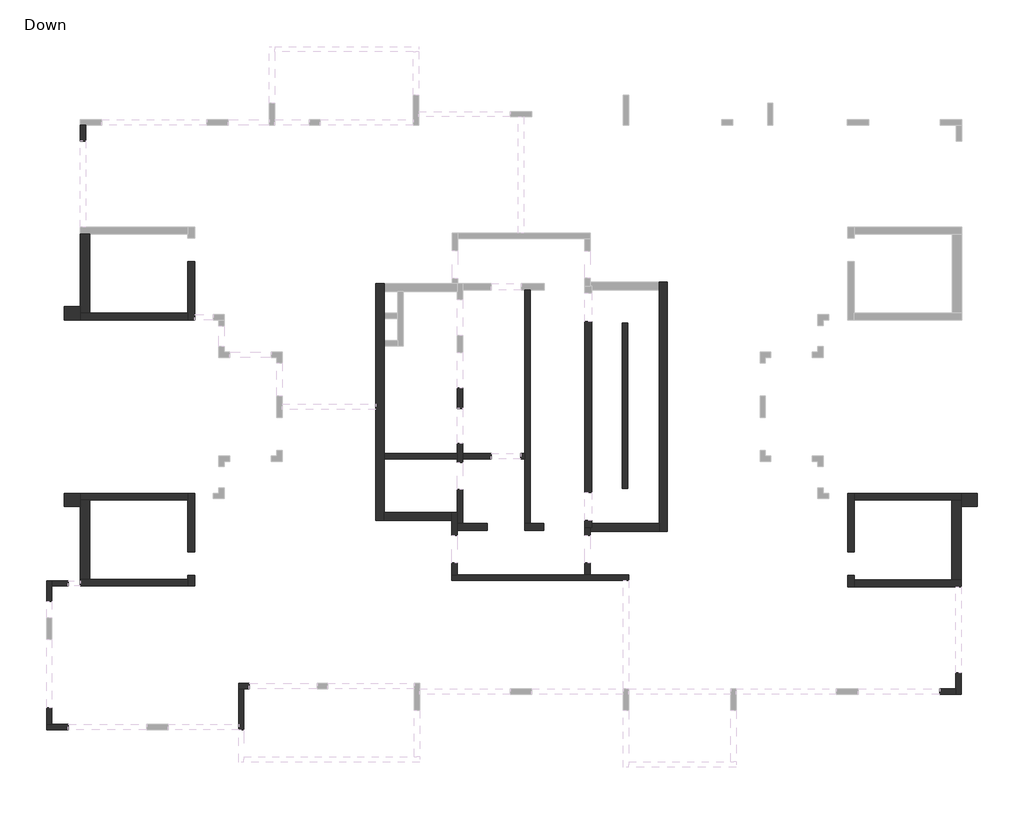
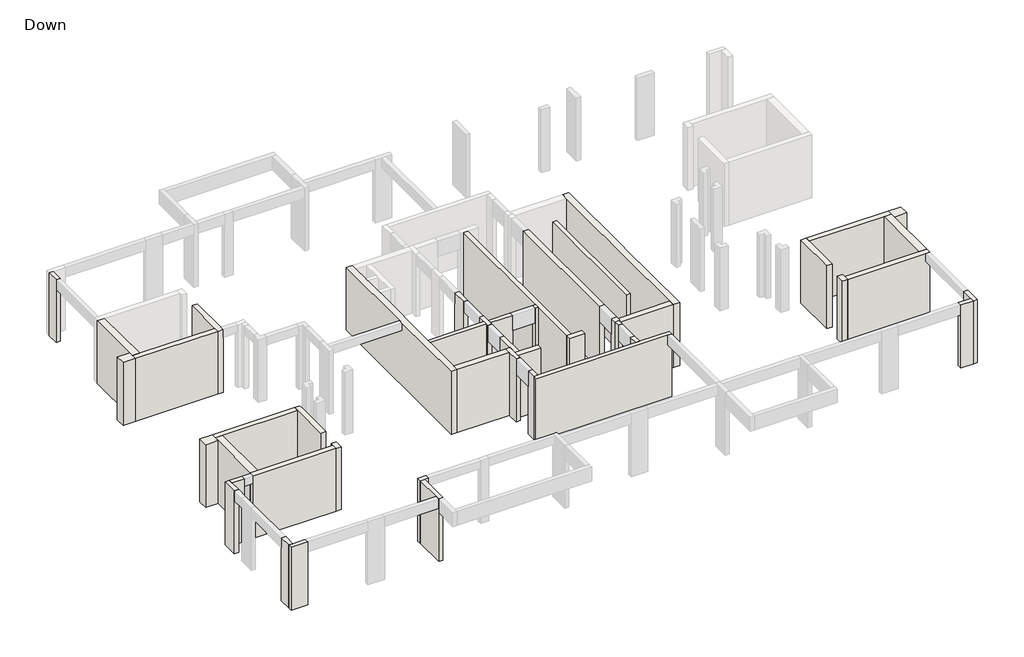
# One storey, part 1 of 3: 46 walls.
"""IFC4 building model written with IfcOpenShell, lengths in millimetres."""

from ifc_helpers import new_model, si_unit, origin, origin_with_axes, place, context, project, spatial, polyline, outline, extrude, faceted_brep, element, save

model = new_model("IFC4")

# Units and contexts
model_context = context("Model", 3, world=origin())
ifc_project = project(units=[si_unit("LENGTHUNIT", "METRE", prefix="MILLI")], contexts=[model_context])

# Site, building, storey
site = spatial("IfcSite", under=ifc_project)
building = spatial("IfcBuilding", under=site)
storey = spatial("IfcBuildingStorey", under=building, Name="Down", Elevation=0.0)

# Walls
placement = place(None, origin())
element("IfcWall", 1, ObjectType="20", at=placement, inside=storey, context=model_context, shape_type="Brep", body=[
    faceted_brep([(-16152.3851738, 8714.1448811, 0.0), (-16152.3851738, 8125.9123109, 0.0), (-16152.3851738, 8125.9123109, 2700.0), (-16152.3851738, 8125.9123109, 3200.0), (-16152.3851738, 8714.1448811, 3200.0), (-15952.3851738, 8714.1448811, 0.0), (-15952.3851738, 8714.1448811, 3020.0), (-15952.3851738, 8714.1448811, 3200.0), (-15952.3851738, 8125.9123109, 3200.0), (-15952.3851738, 8125.9123109, 2700.0), (-15952.3851738, 8125.9123109, 0.0)], [[[0, 1, 2, 3, 4]], [[5, 6, 7, 8, 9, 10]], [[1, 0, 5, 10]], [[3, 2, 1, 10, 9, 8]], [[4, 3, 8, 7]], [[0, 4, 7, 6, 5]]]),
])
element("IfcWall", 2, ObjectType="20", at=placement, inside=storey, context=model_context, shape_type="Brep", body=[
    faceted_brep([(-2227.8189264, -1013.9530422, 0.0), (-2227.8189264, -1753.9530422, 0.0), (-2227.8189264, -1753.9530422, 2670.0), (-2227.8189264, -1753.9530422, 3200.0), (-2227.8189264, -1013.9530422, 3200.0), (-2227.8189264, -1013.9530422, 2670.0), (-2027.8189264, -1013.9530422, 0.0), (-2027.8189264, -1013.9530422, 2670.0), (-2027.8189264, -1013.9530422, 3020.0), (-2027.8189264, -1013.9530422, 3200.0), (-2027.8189264, -1753.9530422, 3200.0), (-2027.8189264, -1753.9530422, 3020.0), (-2027.8189264, -1753.9530422, 2670.0), (-2027.8189264, -1753.9530422, 0.0), (-2032.8189264, -1753.9530422, 3200.0), (-2032.8189264, -1013.9530422, 3200.0)], [[[0, 1, 2, 3, 4, 5]], [[6, 7, 8, 9, 10, 11, 12, 13]], [[1, 0, 6, 13]], [[3, 2, 1, 13, 12, 11, 10, 14]], [[4, 3, 14, 10, 9, 15]], [[0, 5, 4, 15, 9, 8, 7, 6]]]),
])
element("IfcWall", 3, ObjectType="20", at=placement, inside=storey, context=model_context, shape_type="Brep", body=[
    faceted_brep([(-2227.8189264, -3053.9530422, 0.0), (-2227.8189264, -3433.9530422, 0.0), (-2227.8189264, -3633.9530422, 0.0), (-2227.8189264, -3753.9530422, 0.0), (-2227.8189264, -3753.9530422, 2420.0), (-2227.8189264, -3753.9530422, 3200.0), (-2227.8189264, -3633.9530422, 3200.0), (-2227.8189264, -3433.9530422, 3200.0), (-2227.8189264, -3053.9530422, 3200.0), (-2227.8189264, -3053.9530422, 2670.0), (-2027.8189264, -3053.9530422, 0.0), (-2027.8189264, -3053.9530422, 2670.0), (-2027.8189264, -3053.9530422, 3020.0), (-2027.8189264, -3053.9530422, 3200.0), (-2027.8189264, -3433.9530422, 3200.0), (-2027.8189264, -3633.9530422, 3200.0), (-2027.8189264, -3753.9530422, 3200.0), (-2027.8189264, -3753.9530422, 2420.0), (-2027.8189264, -3753.9530422, 0.0), (-2027.8189264, -3633.9530422, 0.0), (-2027.8189264, -3433.9530422, 0.0), (-2032.8189264, -3053.9530422, 3200.0)], [[[0, 1, 2, 3, 4, 5, 6, 7, 8, 9]], [[10, 11, 12, 13, 14, 15, 16, 17, 18, 19, 20]], [[3, 2, 1, 0, 10, 20, 19, 18]], [[5, 4, 3, 18, 17, 16]], [[8, 7, 6, 5, 16, 15, 14, 13, 21]], [[0, 9, 8, 21, 13, 12, 11, 10]]]),
])
element("IfcWall", 4, ObjectType="20", at=placement, inside=storey, context=model_context, shape_type="Brep", body=[
    faceted_brep([(-2027.8189264, -3633.9530422, 0.0), (-967.8189264, -3633.9530422, 0.0), (-967.8189264, -3633.9530422, 2420.0), (-967.8189264, -3633.9530422, 3200.0), (-2027.8189264, -3633.9530422, 3200.0), (-2027.8189264, -3633.9530422, 3020.0), (-2027.8189264, -3433.9530422, 0.0), (-2027.8189264, -3433.9530422, 3020.0), (-2027.8189264, -3433.9530422, 3200.0), (-967.8189264, -3433.9530422, 3200.0), (-967.8189264, -3433.9530422, 2420.0), (-967.8189264, -3433.9530422, 0.0)], [[[0, 1, 2, 3, 4, 5]], [[6, 7, 8, 9, 10, 11]], [[1, 0, 6, 11]], [[3, 2, 1, 11, 10, 9]], [[4, 3, 9, 8]], [[0, 5, 4, 8, 7, 6]]]),
])
element("IfcWall", 5, ObjectType="20", at=placement, inside=storey, context=model_context, shape_type="SweptSolid", body=[
    extrude(outline(polyline([(-4927.8189264, -3433.9530422), (-2227.8189264, -3433.9530422), (-2227.8189264, -3633.9530422), (-4927.8189264, -3633.9530422), (-4927.8189264, -3433.9530422)])), origin_with_axes(), (0.0, 0.0, 1.0), 3200.0),
])
element("IfcWall", 6, ObjectType="20", at=placement, inside=storey, context=model_context, shape_type="Brep", body=[
    faceted_brep([(272.1810736, -3433.9530422, 0.0), (122.0171251, -3433.9530422, 0.0), (122.0171251, -3433.9530422, 2420.0), (122.0171251, -3433.9530422, 3200.0), (272.1810736, -3433.9530422, 3200.0), (272.1810736, -3633.9530422, 0.0), (272.1810736, -3633.9530422, 3020.0), (272.1810736, -3633.9530422, 3200.0), (122.0171251, -3633.9530422, 3200.0), (122.0171251, -3633.9530422, 2420.0), (122.0171251, -3633.9530422, 0.0)], [[[0, 1, 2, 3, 4]], [[5, 6, 7, 8, 9, 10]], [[1, 0, 5, 10]], [[3, 2, 1, 10, 9, 8]], [[4, 3, 8, 7]], [[0, 4, 7, 6, 5]]]),
])
element("IfcWall", 7, ObjectType="20", at=placement, inside=storey, context=model_context, shape_type="Brep", body=[
    faceted_brep([(472.1810736, -6018.9082421, 0.0), (472.1810736, 2608.8247791, 0.0), (472.1810736, 2608.8247791, 3020.0), (472.1810736, 2608.8247791, 3200.0), (472.1810736, -6018.9082421, 3200.0), (472.1810736, -6018.9082421, 3020.0), (272.1810736, -6018.9082421, 0.0), (272.1810736, -6018.9082421, 3200.0), (272.1810736, -3633.9530422, 3200.0), (272.1810736, -3433.9530422, 3200.0), (272.1810736, 2608.8247791, 3200.0), (272.1810736, 2608.8247791, 3020.0), (272.1810736, 2608.8247791, 0.0), (272.1810736, -3433.9530422, 0.0), (272.1810736, -3633.9530422, 0.0)], [[[0, 1, 2, 3, 4, 5]], [[6, 7, 8, 9, 10, 11, 12, 13, 14]], [[1, 0, 6, 14, 13, 12]], [[4, 3, 10, 9, 8, 7]], [[3, 2, 1, 12, 11, 10]], [[0, 5, 4, 7, 6]]]),
])
element("IfcWall", 8, ObjectType="20", at=placement, inside=storey, context=model_context, shape_type="SweptSolid", body=[
    extrude(outline(polyline([(4072.1544873, 1402.9570331), (4072.1544873, -4717.0429669), (3872.1544873, -4717.0429669), (3872.1544873, 1402.9570331), (4072.1544873, 1402.9570331)])), origin_with_axes(), (0.0, 0.0, 1.0), 3200.0),
])
element("IfcWall", 9, ObjectType="20", at=placement, inside=storey, context=model_context, shape_type="Brep", body=[
    faceted_brep([(2484.725333, -6161.1752209, 0.0), (2484.725333, -6451.1752209, 0.0), (2484.725333, -6451.1752209, 2420.0), (2484.725333, -6451.1752209, 3200.0), (2484.725333, -6161.1752209, 3200.0), (2684.725333, -6161.1752209, 0.0), (2684.725333, -6161.1752209, 3200.0), (2684.725333, -6311.1752209, 3200.0), (2684.725333, -6451.1752209, 3200.0), (2684.725333, -6451.1752209, 2420.0), (2684.725333, -6451.1752209, 0.0), (2684.725333, -6311.1752209, 0.0)], [[[0, 1, 2, 3, 4]], [[5, 6, 7, 8, 9, 10, 11]], [[1, 0, 5, 11, 10]], [[3, 2, 1, 10, 9, 8]], [[4, 3, 8, 7, 6]], [[0, 4, 6, 5]]]),
])
element("IfcWall", 10, ObjectType="20", at=placement, inside=storey, context=model_context, shape_type="Brep", body=[
    faceted_brep([(2484.725333, -7471.1752209, 0.0), (2484.725333, -7911.1752209, 0.0), (2484.725333, -7911.1752209, 3020.0), (2484.725333, -7911.1752209, 3200.0), (2484.725333, -7471.1752209, 3200.0), (2484.725333, -7471.1752209, 2420.0), (2684.725333, -7471.1752209, 0.0), (2684.725333, -7471.1752209, 2420.0), (2684.725333, -7471.1752209, 3200.0), (2684.725333, -7911.1752209, 3200.0), (2684.725333, -7911.1752209, 3020.0), (2684.725333, -7911.1752209, 0.0)], [[[0, 1, 2, 3, 4, 5]], [[6, 7, 8, 9, 10, 11]], [[1, 0, 6, 11]], [[4, 3, 9, 8]], [[0, 5, 4, 8, 7, 6]], [[3, 2, 1, 11, 10, 9]]]),
])
element("IfcWall", 11, ObjectType="20", at=placement, inside=storey, context=model_context, shape_type="Brep", body=[
    faceted_brep([(4107.8539459, -7911.1752209, 0.0), (2684.725333, -7911.1752209, 0.0), (2484.725333, -7911.1752209, 0.0), (-2224.4804119, -7911.1752209, 0.0), (-2424.4804119, -7911.1752209, 0.0), (-2424.4804119, -7911.1752209, 3200.0), (-2224.4804119, -7911.1752209, 3200.0), (2484.725333, -7911.1752209, 3200.0), (2684.725333, -7911.1752209, 3200.0), (4107.8539459, -7911.1752209, 3200.0), (4107.8539459, -7911.1752209, 3020.0), (4107.8539459, -8111.1752209, 0.0), (4107.8539459, -8111.1752209, 3200.0), (3907.8539459, -8111.1752209, 3200.0), (-2424.4804119, -8111.1752209, 3200.0), (-2424.4804119, -8111.1752209, 3020.0), (-2424.4804119, -8111.1752209, 0.0)], [[[0, 1, 2, 3, 4, 5, 6, 7, 8, 9, 10]], [[11, 12, 13, 14, 15, 16]], [[4, 3, 2, 1, 0, 11, 16]], [[9, 8, 7, 6, 5, 14, 13, 12]], [[0, 10, 9, 12, 11]], [[5, 4, 16, 15, 14]]]),
])
element("IfcWall", 12, ObjectType="20", at=placement, inside=storey, context=model_context, shape_type="Brep", body=[
    faceted_brep([(-2224.4804119, -7911.1752209, 0.0), (-2224.4804119, -7466.1752209, 0.0), (-2224.4804119, -7466.1752209, 2420.0), (-2224.4804119, -7466.1752209, 3200.0), (-2224.4804119, -7911.1752209, 3200.0), (-2224.4804119, -7911.1752209, 3020.0), (-2424.4804119, -7911.1752209, 0.0), (-2424.4804119, -7911.1752209, 3200.0), (-2424.4804119, -7466.1752209, 3200.0), (-2424.4804119, -7466.1752209, 2420.0), (-2424.4804119, -7466.1752209, 0.0)], [[[0, 1, 2, 3, 4, 5]], [[6, 7, 8, 9, 10]], [[1, 0, 6, 10]], [[3, 2, 1, 10, 9, 8]], [[4, 3, 8, 7]], [[0, 5, 4, 7, 6]]]),
])
element("IfcWall", 13, ObjectType="20", at=placement, inside=storey, context=model_context, shape_type="Brep", body=[
    faceted_brep([(-2224.4804119, -6461.1752209, 0.0), (-2224.4804119, -6261.1752209, 0.0), (-2224.4804119, -6011.1752209, 0.0), (-2224.4804119, -5601.1752209, 0.0), (-2224.4804119, -5601.1752209, 3200.0), (-2224.4804119, -6011.1752209, 3200.0), (-2224.4804119, -6261.1752209, 3200.0), (-2224.4804119, -6461.1752209, 3200.0), (-2224.4804119, -6461.1752209, 2420.0), (-2424.4804119, -6461.1752209, 0.0), (-2424.4804119, -6461.1752209, 2420.0), (-2424.4804119, -6461.1752209, 3200.0), (-2424.4804119, -5901.1752209, 3200.0), (-2424.4804119, -5601.1752209, 3200.0), (-2424.4804119, -5601.1752209, 0.0), (-2424.4804119, -5901.1752209, 0.0), (-2227.8189264, -5601.1752209, 0.0), (-2227.8189264, -5601.1752209, 3200.0)], [[[0, 1, 2, 3, 4, 5, 6, 7, 8]], [[9, 10, 11, 12, 13, 14, 15]], [[3, 2, 1, 0, 9, 15, 14, 16]], [[7, 6, 5, 4, 17, 13, 12, 11]], [[0, 8, 7, 11, 10, 9]], [[4, 3, 16, 14, 13, 17]]]),
])
element("IfcWall", 14, ObjectType="20", at=placement, inside=storey, context=model_context, shape_type="Brep", body=[
    faceted_brep([(-2227.8189264, -4756.1752209, 3200.0), (-2227.8189264, -4756.1752209, 2420.0), (-2227.8189264, -4756.1752209, 0.0), (-2227.8189264, -5601.1752209, 0.0), (-2227.8189264, -5601.1752209, 3200.0), (-2027.8189264, -6011.1752209, 0.0), (-2027.8189264, -4756.1752209, 0.0), (-2027.8189264, -4756.1752209, 2420.0), (-2027.8189264, -4756.1752209, 3200.0), (-2027.8189264, -6011.1752209, 3200.0), (-2027.8189264, -6011.1752209, 3020.0), (-2224.4804119, -6011.1752209, 0.0), (-2224.4804119, -5601.1752209, 0.0), (-2224.4804119, -5601.1752209, 3200.0), (-2224.4804119, -6011.1752209, 3200.0)], [[[0, 1, 2, 3, 4]], [[5, 6, 7, 8, 9, 10]], [[6, 5, 11, 12, 3, 2]], [[9, 8, 0, 4, 13, 14]], [[2, 1, 0, 8, 7, 6]], [[5, 10, 9, 14, 11]], [[13, 12, 11, 14]], [[12, 13, 4, 3]]]),
])
element("IfcWall", 15, ObjectType="20", at=placement, inside=storey, context=model_context, shape_type="Brep", body=[
    faceted_brep([(16190.4478267, -11524.2691374, 0.0), (16190.4478267, -12124.2691374, 0.0), (16190.4478267, -12324.2691374, 0.0), (16190.4478267, -12324.2691374, 3200.0), (16190.4478267, -12124.2691374, 3200.0), (16190.4478267, -11524.2691374, 3200.0), (16190.4478267, -11524.2691374, 2800.0), (16390.4478267, -11524.2691374, 0.0), (16390.4478267, -11524.2691374, 2800.0), (16390.4478267, -11524.2691374, 3200.0), (16390.4478267, -12324.2691374, 3200.0), (16390.4478267, -12324.2691374, 0.0)], [[[0, 1, 2, 3, 4, 5, 6]], [[7, 8, 9, 10, 11]], [[2, 1, 0, 7, 11]], [[5, 4, 3, 10, 9]], [[0, 6, 5, 9, 8, 7]], [[3, 2, 11, 10]]]),
])
element("IfcWall", 16, ObjectType="20", at=placement, inside=storey, context=model_context, shape_type="Brep", body=[
    faceted_brep([(16190.4478267, -12124.2691374, 0.0), (15592.9268131, -12124.2691374, 0.0), (15592.9268131, -12124.2691374, 2700.0), (15592.9268131, -12124.2691374, 3200.0), (16190.4478267, -12124.2691374, 3200.0), (16190.4478267, -12124.2691374, 3020.0), (16190.4478267, -12324.2691374, 0.0), (16190.4478267, -12324.2691374, 3200.0), (15592.9268131, -12324.2691374, 3200.0), (15592.9268131, -12324.2691374, 2700.0), (15592.9268131, -12324.2691374, 0.0)], [[[0, 1, 2, 3, 4, 5]], [[6, 7, 8, 9, 10]], [[1, 0, 6, 10]], [[3, 2, 1, 10, 9, 8]], [[4, 3, 8, 7]], [[0, 5, 4, 7, 6]]]),
])
element("IfcWall", 17, ObjectType="20", at=placement, inside=storey, context=model_context, shape_type="Brep", body=[
    faceted_brep([(-9913.9547043, -11921.300832, 0.0), (-10303.9547043, -11921.300832, 0.0), (-10303.9547043, -11921.300832, 3020.0), (-10303.9547043, -11921.300832, 3200.0), (-9913.9547043, -11921.300832, 3200.0), (-9913.9547043, -11921.300832, 2800.0), (-9913.9547043, -12121.300832, 0.0), (-9913.9547043, -12121.300832, 2800.0), (-9913.9547043, -12121.300832, 3200.0), (-10103.9547043, -12121.300832, 3200.0), (-10303.9547043, -12121.300832, 3200.0), (-10303.9547043, -12121.300832, 0.0), (-10103.9547043, -12121.300832, 0.0)], [[[0, 1, 2, 3, 4, 5]], [[6, 7, 8, 9, 10, 11, 12]], [[1, 0, 6, 12, 11]], [[4, 3, 10, 9, 8]], [[0, 5, 4, 8, 7, 6]], [[3, 2, 1, 11, 10]]]),
])
element("IfcWall", 18, ObjectType="20", at=placement, inside=storey, context=model_context, shape_type="Brep", body=[
    faceted_brep([(-10303.9547043, -12121.300832, 0.0), (-10303.9547043, -13632.1139628, 0.0), (-10303.9547043, -13632.1139628, 2500.0), (-10303.9547043, -13632.1139628, 3200.0), (-10303.9547043, -13432.1139628, 3200.0), (-10303.9547043, -12121.300832, 3200.0), (-10103.9547043, -12121.300832, 0.0), (-10103.9547043, -12121.300832, 3020.0), (-10103.9547043, -12121.300832, 3200.0), (-10103.9547043, -13632.1139628, 3200.0), (-10103.9547043, -13632.1139628, 2500.0), (-10103.9547043, -13632.1139628, 0.0)], [[[0, 1, 2, 3, 4, 5]], [[6, 7, 8, 9, 10, 11]], [[1, 0, 6, 11]], [[3, 2, 1, 11, 10, 9]], [[5, 4, 3, 9, 8]], [[0, 5, 8, 7, 6]]]),
])
element("IfcWall", 19, ObjectType="20", at=placement, inside=storey, context=model_context, shape_type="Brep", body=[
    faceted_brep([(-16594.74029, -13432.1139628, 0.0), (-17194.74029, -13432.1139628, 0.0), (-17394.74029, -13432.1139628, 0.0), (-17394.74029, -13432.1139628, 3200.0), (-17194.74029, -13432.1139628, 3200.0), (-16594.74029, -13432.1139628, 3200.0), (-16594.74029, -13432.1139628, 2700.0), (-16594.74029, -13632.1139628, 0.0), (-16594.74029, -13632.1139628, 2700.0), (-16594.74029, -13632.1139628, 3200.0), (-17394.74029, -13632.1139628, 3200.0), (-17394.74029, -13632.1139628, 0.0)], [[[0, 1, 2, 3, 4, 5, 6]], [[7, 8, 9, 10, 11]], [[2, 1, 0, 7, 11]], [[5, 4, 3, 10, 9]], [[0, 6, 5, 9, 8, 7]], [[3, 2, 11, 10]]]),
])
element("IfcWall", 20, ObjectType="20", at=placement, inside=storey, context=model_context, shape_type="Brep", body=[
    faceted_brep([(-17194.74029, -13432.1139628, 0.0), (-17194.74029, -12822.7787814, 0.0), (-17194.74029, -12822.7787814, 2700.0), (-17194.74029, -12822.7787814, 3200.0), (-17194.74029, -13432.1139628, 3200.0), (-17194.74029, -13432.1139628, 3020.0), (-17394.74029, -13432.1139628, 0.0), (-17394.74029, -13432.1139628, 3200.0), (-17394.74029, -12822.7787814, 3200.0), (-17394.74029, -12822.7787814, 2700.0), (-17394.74029, -12822.7787814, 0.0)], [[[0, 1, 2, 3, 4, 5]], [[6, 7, 8, 9, 10]], [[1, 0, 6, 10]], [[3, 2, 1, 10, 9, 8]], [[4, 3, 8, 7]], [[0, 5, 4, 7, 6]]]),
])
element("IfcWall", 21, ObjectType="20", at=placement, inside=storey, context=model_context, shape_type="Brep", body=[
    faceted_brep([(-17194.74029, -8893.4441313, 0.0), (-17194.74029, -8327.5852261, 0.0), (-17194.74029, -8127.5852261, 0.0), (-17194.74029, -8127.5852261, 3200.0), (-17194.74029, -8327.5852261, 3200.0), (-17194.74029, -8893.4441313, 3200.0), (-17194.74029, -8893.4441313, 2700.0), (-17394.74029, -8893.4441313, 0.0), (-17394.74029, -8893.4441313, 2700.0), (-17394.74029, -8893.4441313, 3200.0), (-17394.74029, -8127.5852261, 3200.0), (-17394.74029, -8127.5852261, 0.0)], [[[0, 1, 2, 3, 4, 5, 6]], [[7, 8, 9, 10, 11]], [[2, 1, 0, 7, 11]], [[5, 4, 3, 10, 9]], [[0, 6, 5, 9, 8, 7]], [[3, 2, 11, 10]]]),
])
element("IfcWall", 22, ObjectType="20", at=placement, inside=storey, context=model_context, shape_type="Brep", body=[
    faceted_brep([(-17194.74029, -8327.5852261, 0.0), (-16589.4316206, -8327.5852261, 0.0), (-16589.4316206, -8327.5852261, 2800.0), (-16589.4316206, -8327.5852261, 3200.0), (-17194.74029, -8327.5852261, 3200.0), (-17194.74029, -8327.5852261, 3020.0), (-17194.74029, -8127.5852261, 0.0), (-17194.74029, -8127.5852261, 3200.0), (-16589.4316206, -8127.5852261, 3200.0), (-16589.4316206, -8127.5852261, 2800.0), (-16589.4316206, -8127.5852261, 0.0)], [[[0, 1, 2, 3, 4, 5]], [[6, 7, 8, 9, 10]], [[1, 0, 6, 10]], [[3, 2, 1, 10, 9, 8]], [[4, 3, 8, 7]], [[0, 5, 4, 7, 6]]]),
])
element("IfcWall", 23, ObjectType="25", at=placement, inside=storey, context=model_context, shape_type="Brep", body=[
    faceted_brep([(-12179.8186713, 3668.3687969, 0.0), (-12179.8186713, 1755.2784849, 0.0), (-12179.8186713, 1505.2784849, 0.0), (-12179.8186713, 1505.2784849, 3200.0), (-12179.8186713, 1755.2784849, 3200.0), (-12179.8186713, 3668.3687969, 3200.0), (-12179.8186713, 3668.3687969, 3020.0), (-11929.8186713, 3668.3687969, 0.0), (-11929.8186713, 3668.3687969, 3020.0), (-11929.8186713, 3668.3687969, 3200.0), (-11929.8186713, 1705.2784849, 3200.0), (-11929.8186713, 1505.2784849, 3200.0), (-11929.8186713, 1505.2784849, 2800.0), (-11929.8186713, 1505.2784849, 0.0)], [[[0, 1, 2, 3, 4, 5, 6]], [[7, 8, 9, 10, 11, 12, 13]], [[2, 1, 0, 7, 13]], [[5, 4, 3, 11, 10, 9]], [[0, 6, 5, 9, 8, 7]], [[3, 2, 13, 12, 11]]]),
])
element("IfcWall", 24, ObjectType="25", at=placement, inside=storey, context=model_context, shape_type="Brep", body=[
    faceted_brep([(-12179.8186713, 1755.2784849, 0.0), (-15802.3851738, 1755.2784849, 0.0), (-16152.3851738, 1755.2784849, 0.0), (-16152.3851738, 1755.2784849, 3200.0), (-15802.3851738, 1755.2784849, 3200.0), (-12179.8186713, 1755.2784849, 3200.0), (-12179.8186713, 1755.2784849, 3020.0), (-12179.8186713, 1505.2784849, 0.0), (-12179.8186713, 1505.2784849, 3200.0), (-16152.3851738, 1505.2784849, 3200.0), (-16152.3851738, 1505.2784849, 0.0)], [[[0, 1, 2, 3, 4, 5, 6]], [[7, 8, 9, 10]], [[2, 1, 0, 7, 10]], [[5, 4, 3, 9, 8]], [[0, 6, 5, 8, 7]], [[3, 2, 10, 9]]]),
])
element("IfcWall", 25, ObjectType="25", at=placement, inside=storey, context=model_context, shape_type="Brep", body=[
    faceted_brep([(2484.725333, -5901.1752209, 0.0), (2484.725333, -6161.1752209, 0.0), (2484.725333, -6161.1752209, 3200.0), (2484.725333, -5901.1752209, 3200.0), (2484.725333, -5901.1752209, 2420.0), (2734.725333, -5901.1752209, 0.0), (2734.725333, -5901.1752209, 2420.0), (2734.725333, -5901.1752209, 3200.0), (2734.725333, -6011.1752209, 3200.0), (2734.725333, -6161.1752209, 3200.0), (2734.725333, -6161.1752209, 0.0), (2734.725333, -6011.1752209, 0.0), (2684.725333, -6161.1752209, 0.0), (2684.725333, -6161.1752209, 3200.0)], [[[0, 1, 2, 3, 4]], [[5, 6, 7, 8, 9, 10, 11]], [[1, 0, 5, 11, 10, 12]], [[2, 1, 12, 10, 9, 13]], [[3, 2, 13, 9, 8, 7]], [[0, 4, 3, 7, 6, 5]]]),
])
element("IfcWall", 26, ObjectType="25", at=placement, inside=storey, context=model_context, shape_type="Brep", body=[
    faceted_brep([(-12179.8186713, -8077.5852261, 0.0), (-15802.3851738, -8077.5852261, 0.0), (-16152.3851738, -8077.5852261, 0.0), (-16152.3851738, -8077.5852261, 3200.0), (-15802.3851738, -8077.5852261, 3200.0), (-12179.8186713, -8077.5852261, 3200.0), (-12179.8186713, -8077.5852261, 3020.0), (-12179.8186713, -8327.5852261, 0.0), (-12179.8186713, -8327.5852261, 3200.0), (-16152.3851738, -8327.5852261, 3200.0), (-16152.3851738, -8327.5852261, 2800.0), (-16152.3851738, -8327.5852261, 0.0), (-16152.3851738, -8127.5852261, 3200.0)], [[[0, 1, 2, 3, 4, 5, 6]], [[7, 8, 9, 10, 11]], [[2, 1, 0, 7, 11]], [[5, 4, 3, 12, 9, 8]], [[0, 6, 5, 8, 7]], [[3, 2, 11, 10, 9, 12]]]),
])
element("IfcWall", 27, ObjectType="25", at=placement, inside=storey, context=model_context, shape_type="Brep", body=[
    faceted_brep([(-11929.8186713, -8327.5852261, 0.0), (-11929.8186713, -7927.5852261, 0.0), (-11929.8186713, -7927.5852261, 3020.0), (-11929.8186713, -7927.5852261, 3200.0), (-11929.8186713, -8327.5852261, 3200.0), (-11929.8186713, -8327.5852261, 3020.0), (-12179.8186713, -8327.5852261, 0.0), (-12179.8186713, -8327.5852261, 3200.0), (-12179.8186713, -8077.5852261, 3200.0), (-12179.8186713, -7927.5852261, 3200.0), (-12179.8186713, -7927.5852261, 3020.0), (-12179.8186713, -7927.5852261, 0.0), (-12179.8186713, -8077.5852261, 0.0)], [[[0, 1, 2, 3, 4, 5]], [[6, 7, 8, 9, 10, 11, 12]], [[1, 0, 6, 12, 11]], [[3, 2, 1, 11, 10, 9]], [[4, 3, 9, 8, 7]], [[0, 5, 4, 7, 6]]]),
])
element("IfcWall", 28, ObjectType="25", at=placement, inside=storey, context=model_context, shape_type="Brep", body=[
    faceted_brep([(-11929.8186713, -7056.2748812, 0.0), (-11929.8186713, -4893.1845693, 0.0), (-11929.8186713, -4893.1845693, 2800.0), (-11929.8186713, -4893.1845693, 3200.0), (-11929.8186713, -5093.1845693, 3200.0), (-11929.8186713, -7056.2748812, 3200.0), (-11929.8186713, -7056.2748812, 3020.0), (-12179.8186713, -7056.2748812, 0.0), (-12179.8186713, -7056.2748812, 3020.0), (-12179.8186713, -7056.2748812, 3200.0), (-12179.8186713, -5143.1845693, 3200.0), (-12179.8186713, -4893.1845693, 3200.0), (-12179.8186713, -4893.1845693, 0.0), (-12179.8186713, -5143.1845693, 0.0)], [[[0, 1, 2, 3, 4, 5, 6]], [[7, 8, 9, 10, 11, 12, 13]], [[1, 0, 7, 13, 12]], [[5, 4, 3, 11, 10, 9]], [[0, 6, 5, 9, 8, 7]], [[3, 2, 1, 12, 11]]]),
])
element("IfcWall", 29, ObjectType="25", at=placement, inside=storey, context=model_context, shape_type="Brep", body=[
    faceted_brep([(-12179.8186713, -4893.1845693, 0.0), (-16152.3851738, -4893.1845693, 0.0), (-16152.3851738, -4893.1845693, 3200.0), (-12179.8186713, -4893.1845693, 3200.0), (-12179.8186713, -5143.1845693, 0.0), (-12179.8186713, -5143.1845693, 3020.0), (-12179.8186713, -5143.1845693, 3200.0), (-15802.3851738, -5143.1845693, 3200.0), (-16152.3851738, -5143.1845693, 3200.0), (-16152.3851738, -5143.1845693, 0.0), (-15802.3851738, -5143.1845693, 0.0)], [[[0, 1, 2, 3]], [[4, 5, 6, 7, 8, 9, 10]], [[1, 0, 4, 10, 9]], [[3, 2, 8, 7, 6]], [[0, 3, 6, 5, 4]], [[2, 1, 9, 8]]]),
])
element("IfcWall", 30, ObjectType="25", at=placement, inside=storey, context=model_context, shape_type="Brep", body=[
    faceted_brep([(12437.8813243, -8347.5852261, 0.0), (16390.4478267, -8347.5852261, 0.0), (16390.4478267, -8347.5852261, 2800.0), (16390.4478267, -8347.5852261, 3200.0), (16190.4478267, -8347.5852261, 3200.0), (12437.8813243, -8347.5852261, 3200.0), (12437.8813243, -8097.5852261, 0.0), (12437.8813243, -8097.5852261, 3020.0), (12437.8813243, -8097.5852261, 3200.0), (16040.4478267, -8097.5852261, 3200.0), (16390.4478267, -8097.5852261, 3200.0), (16390.4478267, -8097.5852261, 0.0), (16040.4478267, -8097.5852261, 0.0)], [[[0, 1, 2, 3, 4, 5]], [[6, 7, 8, 9, 10, 11, 12]], [[1, 0, 6, 12, 11]], [[5, 4, 3, 10, 9, 8]], [[0, 5, 8, 7, 6]], [[3, 2, 1, 11, 10]]]),
])
element("IfcWall", 31, ObjectType="25", at=placement, inside=storey, context=model_context, shape_type="Brep", body=[
    faceted_brep([(12437.8813243, -8347.5852261, 0.0), (12437.8813243, -8097.5852261, 0.0), (12437.8813243, -7927.5852261, 0.0), (12437.8813243, -7927.5852261, 3020.0), (12437.8813243, -7927.5852261, 3200.0), (12437.8813243, -8097.5852261, 3200.0), (12437.8813243, -8347.5852261, 3200.0), (12187.8813243, -8347.5852261, 0.0), (12187.8813243, -8347.5852261, 3020.0), (12187.8813243, -8347.5852261, 3200.0), (12187.8813243, -7927.5852261, 3200.0), (12187.8813243, -7927.5852261, 3020.0), (12187.8813243, -7927.5852261, 0.0)], [[[0, 1, 2, 3, 4, 5, 6]], [[7, 8, 9, 10, 11, 12]], [[2, 1, 0, 7, 12]], [[4, 3, 2, 12, 11, 10]], [[6, 5, 4, 10, 9]], [[0, 6, 9, 8, 7]]]),
])
element("IfcWall", 32, ObjectType="25", at=placement, inside=storey, context=model_context, shape_type="Brep", body=[
    faceted_brep([(12437.8813243, -7056.2748812, 0.0), (12437.8813243, -5143.1845693, 0.0), (12437.8813243, -4893.1845693, 0.0), (12437.8813243, -4893.1845693, 3200.0), (12437.8813243, -5143.1845693, 3200.0), (12437.8813243, -7056.2748812, 3200.0), (12437.8813243, -7056.2748812, 3020.0), (12187.8813243, -7056.2748812, 0.0), (12187.8813243, -7056.2748812, 3020.0), (12187.8813243, -7056.2748812, 3200.0), (12187.8813243, -5093.1845693, 3200.0), (12187.8813243, -4893.1845693, 3200.0), (12187.8813243, -4893.1845693, 2800.0), (12187.8813243, -4893.1845693, 0.0)], [[[0, 1, 2, 3, 4, 5, 6]], [[7, 8, 9, 10, 11, 12, 13]], [[2, 1, 0, 7, 13]], [[5, 4, 3, 11, 10, 9]], [[0, 6, 5, 9, 8, 7]], [[3, 2, 13, 12, 11]]]),
])
element("IfcWall", 33, ObjectType="25", at=placement, inside=storey, context=model_context, shape_type="Brep", body=[
    faceted_brep([(12437.8813243, -5143.1845693, 0.0), (16040.4478267, -5143.1845693, 0.0), (16390.4478267, -5143.1845693, 0.0), (16390.4478267, -5143.1845693, 3200.0), (16040.4478267, -5143.1845693, 3200.0), (12437.8813243, -5143.1845693, 3200.0), (12437.8813243, -5143.1845693, 3020.0), (12437.8813243, -4893.1845693, 0.0), (12437.8813243, -4893.1845693, 3200.0), (16390.4478267, -4893.1845693, 3200.0), (16390.4478267, -4893.1845693, 0.0)], [[[0, 1, 2, 3, 4, 5, 6]], [[7, 8, 9, 10]], [[2, 1, 0, 7, 10]], [[5, 4, 3, 9, 8]], [[0, 6, 5, 8, 7]], [[3, 2, 10, 9]]]),
])
element("IfcWall", 34, ObjectType="25", at=placement, inside=storey, context=model_context, shape_type="Brep", body=[
    faceted_brep([(2484.725333, 1454.2743435, 0.0), (2484.725333, -4865.7256565, 0.0), (2484.725333, -4865.7256565, 2420.0), (2484.725333, -4865.7256565, 3200.0), (2484.725333, 1454.2743435, 3200.0), (2484.725333, 1454.2743435, 2420.0), (2734.725333, 1454.2743435, 0.0), (2734.725333, 1454.2743435, 2420.0), (2734.725333, 1454.2743435, 3200.0), (2734.725333, 1402.9570331, 3200.0), (2734.725333, -4865.7256565, 3200.0), (2734.725333, -4865.7256565, 2420.0), (2734.725333, -4865.7256565, 0.0)], [[[0, 1, 2, 3, 4, 5]], [[6, 7, 8, 9, 10, 11, 12]], [[1, 0, 6, 12]], [[3, 2, 1, 12, 11, 10]], [[4, 3, 10, 9, 8]], [[0, 5, 4, 8, 7, 6]]]),
])
element("IfcWall", 35, ObjectType="25", at=placement, inside=storey, context=model_context, shape_type="Brep", body=[
    faceted_brep([(-2224.4804119, -6261.1752209, 0.0), (-1124.4804119, -6261.1752209, 0.0), (-1124.4804119, -6261.1752209, 3020.0), (-1124.4804119, -6261.1752209, 3200.0), (-2224.4804119, -6261.1752209, 3200.0), (-2224.4804119, -6261.1752209, 3020.0), (-2224.4804119, -6011.1752209, 0.0), (-2224.4804119, -6011.1752209, 3200.0), (-2027.8189264, -6011.1752209, 3200.0), (-1124.4804119, -6011.1752209, 3200.0), (-1124.4804119, -6011.1752209, 3020.0), (-1124.4804119, -6011.1752209, 0.0), (-2027.8189264, -6011.1752209, 0.0)], [[[0, 1, 2, 3, 4, 5]], [[6, 7, 8, 9, 10, 11, 12]], [[1, 0, 6, 12, 11]], [[3, 2, 1, 11, 10, 9]], [[4, 3, 9, 8, 7]], [[0, 5, 4, 7, 6]]]),
])
element("IfcWall", 36, ObjectType="25", at=placement, inside=storey, context=model_context, shape_type="Brep", body=[
    faceted_brep([(974.071657, -6018.9082421, 0.0), (472.1810736, -6018.9082421, 0.0), (272.1810736, -6018.9082421, 0.0), (272.1810736, -6018.9082421, 3200.0), (472.1810736, -6018.9082421, 3200.0), (974.071657, -6018.9082421, 3200.0), (974.071657, -6018.9082421, 3020.0), (974.071657, -6268.9082421, 0.0), (974.071657, -6268.9082421, 3020.0), (974.071657, -6268.9082421, 3200.0), (272.1810736, -6268.9082421, 3200.0), (272.1810736, -6268.9082421, 3020.0), (272.1810736, -6268.9082421, 0.0)], [[[0, 1, 2, 3, 4, 5, 6]], [[7, 8, 9, 10, 11, 12]], [[2, 1, 0, 7, 12]], [[5, 4, 3, 10, 9]], [[0, 6, 5, 9, 8, 7]], [[3, 2, 12, 11, 10]]]),
])
element("IfcWall", 37, ObjectType="30", at=placement, inside=storey, context=model_context, shape_type="Brep", body=[
    faceted_brep([(-5227.8189264, 2858.8247791, 0.0), (-5227.8189264, -5901.1752209, 0.0), (-5227.8189264, -5901.1752209, 3020.0), (-5227.8189264, -5901.1752209, 3200.0), (-5227.8189264, -1793.9530422, 3200.0), (-5227.8189264, -1593.9530422, 3200.0), (-5227.8189264, 2858.8247791, 3200.0), (-5227.8189264, 2858.8247791, 3020.0), (-4927.8189264, 2858.8247791, 0.0), (-4927.8189264, 2858.8247791, 3200.0), (-4927.8189264, 2558.8247791, 3200.0), (-4927.8189264, 1760.873998, 3200.0), (-4927.8189264, 1560.873998, 3200.0), (-4927.8189264, 753.8247791, 3200.0), (-4927.8189264, 553.8247791, 3200.0), (-4927.8189264, -3433.9530422, 3200.0), (-4927.8189264, -3633.9530422, 3200.0), (-4927.8189264, -5601.1752209, 3200.0), (-4927.8189264, -5901.1752209, 3200.0), (-4927.8189264, -5901.1752209, 0.0), (-4927.8189264, -5601.1752209, 0.0), (-4927.8189264, -3633.9530422, 0.0), (-4927.8189264, -3433.9530422, 0.0), (-4927.8189264, 553.8247791, 0.0), (-4927.8189264, 753.8247791, 0.0), (-4927.8189264, 1560.873998, 0.0), (-4927.8189264, 1760.873998, 0.0), (-4927.8189264, 2558.8247791, 0.0)], [[[0, 1, 2, 3, 4, 5, 6, 7]], [[8, 9, 10, 11, 12, 13, 14, 15, 16, 17, 18, 19, 20, 21, 22, 23, 24, 25, 26, 27]], [[1, 0, 8, 27, 26, 25, 24, 23, 22, 21, 20, 19]], [[6, 5, 4, 3, 18, 17, 16, 15, 14, 13, 12, 11, 10, 9]], [[3, 2, 1, 19, 18]], [[0, 7, 6, 9, 8]]]),
])
element("IfcWall", 38, ObjectType="30", at=placement, inside=storey, context=model_context, shape_type="Brep", body=[
    faceted_brep([(-4927.8189264, -5901.1752209, 0.0), (-2424.4804119, -5901.1752209, 0.0), (-2424.4804119, -5901.1752209, 3020.0), (-2424.4804119, -5901.1752209, 3200.0), (-4927.8189264, -5901.1752209, 3200.0), (-4927.8189264, -5601.1752209, 0.0), (-4927.8189264, -5601.1752209, 3200.0), (-2424.4804119, -5601.1752209, 3200.0), (-2424.4804119, -5601.1752209, 0.0)], [[[0, 1, 2, 3, 4]], [[5, 6, 7, 8]], [[1, 0, 5, 8]], [[4, 3, 7, 6]], [[0, 4, 6, 5]], [[3, 2, 1, 8, 7]]]),
])
element("IfcWall", 39, ObjectType="30", at=placement, inside=storey, context=model_context, shape_type="Brep", body=[
    faceted_brep([(5225.8815794, 2916.2932633, 0.0), (5225.8815794, 2616.2932633, 0.0), (5225.8815794, -6011.1752209, 0.0), (5225.8815794, -6311.1752209, 0.0), (5225.8815794, -6311.1752209, 3200.0), (5225.8815794, -6011.1752209, 3200.0), (5225.8815794, 1402.9570331, 3200.0), (5225.8815794, 2616.2932633, 3200.0), (5225.8815794, 2916.2932633, 3200.0), (5525.8815794, 2916.2932633, 0.0), (5525.8815794, 2916.2932633, 3020.0), (5525.8815794, 2916.2932633, 3200.0), (5525.8815794, -1593.9530422, 3200.0), (5525.8815794, -1793.9530422, 3200.0), (5525.8815794, -6311.1752209, 3200.0), (5525.8815794, -6311.1752209, 3020.0), (5525.8815794, -6311.1752209, 0.0)], [[[0, 1, 2, 3, 4, 5, 6, 7, 8]], [[9, 10, 11, 12, 13, 14, 15, 16]], [[3, 2, 1, 0, 9, 16]], [[8, 7, 6, 5, 4, 14, 13, 12, 11]], [[4, 3, 16, 15, 14]], [[0, 8, 11, 10, 9]]]),
])
element("IfcWall", 40, ObjectType="30", at=placement, inside=storey, context=model_context, shape_type="Brep", body=[
    faceted_brep([(5225.8815794, -6011.1752209, 0.0), (2734.725333, -6011.1752209, 0.0), (2734.725333, -6011.1752209, 3200.0), (5225.8815794, -6011.1752209, 3200.0), (5225.8815794, -6311.1752209, 0.0), (5225.8815794, -6311.1752209, 3200.0), (2684.725333, -6311.1752209, 3200.0), (2684.725333, -6311.1752209, 3020.0), (2684.725333, -6311.1752209, 0.0), (2684.725333, -6161.1752209, 0.0), (2734.725333, -6161.1752209, 0.0), (2734.725333, -6161.1752209, 3200.0), (2684.725333, -6161.1752209, 3200.0)], [[[0, 1, 2, 3]], [[4, 5, 6, 7, 8]], [[1, 0, 4, 8, 9, 10]], [[3, 2, 11, 12, 6, 5]], [[0, 3, 5, 4]], [[2, 1, 10, 11]], [[10, 9, 12, 11]], [[9, 8, 7, 6, 12]]]),
])
element("IfcWall", 41, ObjectType="35", at=placement, inside=storey, context=model_context, shape_type="Brep", body=[
    faceted_brep([(-15802.3851738, 1755.2784849, 0.0), (-15802.3851738, 4689.6791417, 0.0), (-15802.3851738, 4689.6791417, 3020.0), (-15802.3851738, 4689.6791417, 3200.0), (-15802.3851738, 1755.2784849, 3200.0), (-15802.3851738, 1755.2784849, 3020.0), (-16152.3851738, 1755.2784849, 0.0), (-16152.3851738, 1755.2784849, 3200.0), (-16152.3851738, 1995.2784849, 3200.0), (-16152.3851738, 4689.6791417, 3200.0), (-16152.3851738, 4689.6791417, 0.0), (-16152.3851738, 1995.2784849, 0.0)], [[[0, 1, 2, 3, 4, 5]], [[6, 7, 8, 9, 10, 11]], [[1, 0, 6, 11, 10]], [[4, 3, 9, 8, 7]], [[0, 5, 4, 7, 6]], [[3, 2, 1, 10, 9]]]),
])
element("IfcWall", 42, ObjectType="35", at=placement, inside=storey, context=model_context, shape_type="Brep", body=[
    faceted_brep([(-16152.3851738, -5143.1845693, 0.0), (-16152.3851738, -5383.1845693, 0.0), (-16152.3851738, -8077.5852261, 0.0), (-16152.3851738, -8077.5852261, 3200.0), (-16152.3851738, -5383.1845693, 3200.0), (-16152.3851738, -5143.1845693, 3200.0), (-15802.3851738, -5143.1845693, 0.0), (-15802.3851738, -5143.1845693, 3020.0), (-15802.3851738, -5143.1845693, 3200.0), (-15802.3851738, -8077.5852261, 3200.0), (-15802.3851738, -8077.5852261, 3020.0), (-15802.3851738, -8077.5852261, 0.0)], [[[0, 1, 2, 3, 4, 5]], [[6, 7, 8, 9, 10, 11]], [[2, 1, 0, 6, 11]], [[5, 4, 3, 9, 8]], [[0, 5, 8, 7, 6]], [[3, 2, 11, 10, 9]]]),
])
element("IfcWall", 43, ObjectType="35", at=placement, inside=storey, context=model_context, shape_type="Brep", body=[
    faceted_brep([(16040.4478267, -5143.1845693, 0.0), (16040.4478267, -8097.5852261, 0.0), (16040.4478267, -8097.5852261, 3020.0), (16040.4478267, -8097.5852261, 3200.0), (16040.4478267, -5143.1845693, 3200.0), (16040.4478267, -5143.1845693, 3020.0), (16390.4478267, -5143.1845693, 0.0), (16390.4478267, -5143.1845693, 3200.0), (16390.4478267, -5383.1845693, 3200.0), (16390.4478267, -8097.5852261, 3200.0), (16390.4478267, -8097.5852261, 0.0), (16390.4478267, -5383.1845693, 0.0)], [[[0, 1, 2, 3, 4, 5]], [[6, 7, 8, 9, 10, 11]], [[1, 0, 6, 11, 10]], [[4, 3, 9, 8, 7]], [[0, 5, 4, 7, 6]], [[3, 2, 1, 10, 9]]]),
])
element("IfcWall", 44, ObjectType="60", at=placement, inside=storey, context=model_context, shape_type="Brep", body=[
    faceted_brep([(-16748.892563, 1995.2784849, 0.0), (-16748.892563, 1505.2784849, 0.0), (-16748.892563, 1505.2784849, 3200.0), (-16748.892563, 1995.2784849, 3200.0), (-16152.3851738, 1995.2784849, 0.0), (-16152.3851738, 1755.2784849, 0.0), (-16152.3851738, 1505.2784849, 0.0), (-16152.3851738, 1995.2784849, 3200.0), (-16152.3851738, 1505.2784849, 3200.0), (-16152.3851738, 1755.2784849, 3200.0)], [[[0, 1, 2, 3]], [[1, 0, 4, 5, 6]], [[0, 3, 7, 4]], [[3, 2, 8, 9, 7]], [[2, 1, 6, 8]], [[4, 7, 9, 8, 6, 5]]]),
])
element("IfcWall", 45, ObjectType="60", at=placement, inside=storey, context=model_context, shape_type="Brep", body=[
    faceted_brep([(-16748.892563, -4893.1845693, 0.0), (-16748.892563, -5383.1845693, 0.0), (-16748.892563, -5383.1845693, 3200.0), (-16748.892563, -4893.1845693, 3200.0), (-16152.3851738, -4893.1845693, 0.0), (-16152.3851738, -5143.1845693, 0.0), (-16152.3851738, -5383.1845693, 0.0), (-16152.3851738, -5383.1845693, 3200.0), (-16152.3851738, -5143.1845693, 3200.0), (-16152.3851738, -4893.1845693, 3200.0)], [[[0, 1, 2, 3]], [[1, 0, 4, 5, 6]], [[2, 1, 6, 7]], [[3, 2, 7, 8, 9]], [[0, 3, 9, 4]], [[4, 9, 8, 7, 6, 5]]]),
])
element("IfcWall", 46, ObjectType="60", at=placement, inside=storey, context=model_context, shape_type="Brep", body=[
    faceted_brep([(16986.9552159, -5383.1845693, 0.0), (16986.9552159, -4893.1845693, 0.0), (16986.9552159, -4893.1845693, 3200.0), (16986.9552159, -5383.1845693, 3200.0), (16390.4478267, -5383.1845693, 0.0), (16390.4478267, -5143.1845693, 0.0), (16390.4478267, -4893.1845693, 0.0), (16390.4478267, -5383.1845693, 3200.0), (16390.4478267, -4893.1845693, 3200.0), (16390.4478267, -5143.1845693, 3200.0)], [[[0, 1, 2, 3]], [[1, 0, 4, 5, 6]], [[0, 3, 7, 4]], [[3, 2, 8, 9, 7]], [[2, 1, 6, 8]], [[4, 7, 9, 8, 6, 5]]]),
])

save(model, "model.ifc")

# Revit data of these elements
# Project information
#   Project Issue Date = "Issue Date"
#   Project Status = "Project Status"
#   Client Name = "לקוח"
#   Project Address = "Enter address here"
#   Project Name = "Project 035"
#   Project Number = "מספר פרויקט"
# Type "20"
#   Layers, outside or top first: 20 cm "Concrete" (function 1)
# Type "25"
#   Layers, outside or top first: 25 cm "Concrete" (function 1)
# Type "30"
#   Layers, outside or top first: 30 cm "Concrete" (function 1)
# Type "35"
#   Layers, outside or top first: 35 cm "Concrete" (function 1)
# Type "60"
#   Layers, outside or top first: 60 cm "Concrete" (function 1)
# Element 1 (IfcWall, "20")
#   Comments = ""
#   Mark = "W2"
#   SOFiSTiK_EdgeZones = "W2"
#   SOFiSTiK_AMG_Comments = ""
#   Top Offset = 0 cm
#   Base Offset = 0 cm
#   wall height = 320 cm
#   SOFiSTiK_AMG_Scheduled = yes
#   SOFiSTiK_AMG_Adjusted = yes
#   Phase Created = New Construction
#   Base Constraint = Down
#   Top Constraint = Typical Floor
#   Materials on its faces: "Concrete"
# Element 2 (IfcWall, "20")
#   Comments = ""
#   Mark = "W27"
#   SOFiSTiK_EdgeZones = "W27"
#   SOFiSTiK_AMG_Comments = ""
#   Top Offset = 0 cm
#   Base Offset = 0 cm
#   wall height = 320 cm
#   SOFiSTiK_AMG_Scheduled = yes
#   SOFiSTiK_AMG_Adjusted = yes
#   Phase Created = New Construction
#   Base Constraint = Down
#   Top Constraint = Typical Floor
#   Materials on its faces: "Concrete"
# Element 3 (IfcWall, "20")
#   Comments = ""
#   Mark = "W28"
#   SOFiSTiK_EdgeZones = "W28"
#   SOFiSTiK_AMG_Comments = ""
#   Top Offset = 0 cm
#   Base Offset = 0 cm
#   wall height = 320 cm
#   SOFiSTiK_AMG_Scheduled = yes
#   SOFiSTiK_AMG_Adjusted = yes
#   Phase Created = New Construction
#   Base Constraint = Down
#   Top Constraint = Typical Floor
#   Materials on its faces: "Concrete"
# Element 4 (IfcWall, "20")
#   Comments = ""
#   Mark = "W29"
#   SOFiSTiK_EdgeZones = "W29"
#   SOFiSTiK_AMG_Comments = ""
#   Top Offset = 0 cm
#   Base Offset = 0 cm
#   wall height = 320 cm
#   SOFiSTiK_AMG_Scheduled = yes
#   SOFiSTiK_AMG_Adjusted = yes
#   Phase Created = New Construction
#   Base Constraint = Down
#   Top Constraint = Typical Floor
#   Materials on its faces: "Concrete"
# Element 5 (IfcWall, "20")
#   Comments = ""
#   Mark = "W30"
#   SOFiSTiK_EdgeZones = "W30"
#   SOFiSTiK_AMG_Comments = ""
#   Top Offset = 0 cm
#   Base Offset = 0 cm
#   wall height = 320 cm
#   SOFiSTiK_AMG_Scheduled = yes
#   SOFiSTiK_AMG_Adjusted = yes
#   Phase Created = New Construction
#   Base Constraint = Down
#   Top Constraint = Typical Floor
#   Materials on its faces: "Concrete"
# Element 6 (IfcWall, "20")
#   Comments = ""
#   Mark = "W31"
#   SOFiSTiK_EdgeZones = "W31"
#   SOFiSTiK_AMG_Comments = ""
#   Top Offset = 0 cm
#   Base Offset = 0 cm
#   wall height = 320 cm
#   SOFiSTiK_AMG_Scheduled = yes
#   SOFiSTiK_AMG_Adjusted = yes
#   Phase Created = New Construction
#   Base Constraint = Down
#   Top Constraint = Typical Floor
#   Materials on its faces: "Concrete"
# Element 7 (IfcWall, "20")
#   Comments = ""
#   Mark = "W32"
#   SOFiSTiK_EdgeZones = "W32"
#   SOFiSTiK_AMG_Comments = ""
#   Top Offset = 0 cm
#   Base Offset = 0 cm
#   wall height = 320 cm
#   SOFiSTiK_AMG_Scheduled = yes
#   SOFiSTiK_AMG_Adjusted = yes
#   Phase Created = New Construction
#   Base Constraint = Down
#   Top Constraint = Typical Floor
#   Materials on its faces: "Concrete"
# Element 8 (IfcWall, "20")
#   Comments = ""
#   Mark = "W45"
#   SOFiSTiK_EdgeZones = "W45"
#   SOFiSTiK_AMG_Comments = ""
#   Top Offset = 0 cm
#   Base Offset = 0 cm
#   wall height = 320 cm
#   SOFiSTiK_AMG_Scheduled = yes
#   SOFiSTiK_AMG_Adjusted = yes
#   Phase Created = New Construction
#   Base Constraint = Down
#   Top Constraint = Typical Floor
#   Materials on its faces: "Concrete"
# Element 9 (IfcWall, "20")
#   Comments = ""
#   Mark = "W46"
#   SOFiSTiK_EdgeZones = "W46"
#   SOFiSTiK_AMG_Comments = ""
#   Top Offset = 0 cm
#   Base Offset = 0 cm
#   wall height = 320 cm
#   SOFiSTiK_AMG_Scheduled = yes
#   SOFiSTiK_AMG_Adjusted = yes
#   Phase Created = New Construction
#   Base Constraint = Down
#   Top Constraint = Typical Floor
#   Materials on its faces: "Concrete"
# Element 10 (IfcWall, "20")
#   Comments = ""
#   Mark = "W47"
#   SOFiSTiK_EdgeZones = "W47"
#   SOFiSTiK_AMG_Comments = ""
#   Top Offset = 0 cm
#   Base Offset = 0 cm
#   wall height = 320 cm
#   SOFiSTiK_AMG_Scheduled = yes
#   SOFiSTiK_AMG_Adjusted = yes
#   Phase Created = New Construction
#   Base Constraint = Down
#   Top Constraint = Typical Floor
#   Materials on its faces: "Concrete"
# Element 11 (IfcWall, "20")
#   Comments = ""
#   Mark = "W48"
#   SOFiSTiK_EdgeZones = "W49"
#   SOFiSTiK_AMG_Comments = ""
#   Top Offset = 0 cm
#   Base Offset = 0 cm
#   wall height = 320 cm
#   SOFiSTiK_AMG_Scheduled = yes
#   SOFiSTiK_AMG_Adjusted = yes
#   Phase Created = New Construction
#   Base Constraint = Down
#   Top Constraint = Typical Floor
#   Materials on its faces: "Concrete"
# Element 12 (IfcWall, "20")
#   Comments = ""
#   Mark = "W49"
#   SOFiSTiK_EdgeZones = "W50"
#   SOFiSTiK_AMG_Comments = ""
#   Top Offset = 0 cm
#   Base Offset = 0 cm
#   wall height = 320 cm
#   SOFiSTiK_AMG_Scheduled = yes
#   SOFiSTiK_AMG_Adjusted = yes
#   Phase Created = New Construction
#   Base Constraint = Down
#   Top Constraint = Typical Floor
#   Materials on its faces: "Concrete"
# Element 13 (IfcWall, "20")
#   Comments = ""
#   Mark = "W50"
#   SOFiSTiK_EdgeZones = "W51"
#   SOFiSTiK_AMG_Comments = ""
#   Top Offset = 0 cm
#   Base Offset = 0 cm
#   wall height = 320 cm
#   SOFiSTiK_AMG_Scheduled = yes
#   SOFiSTiK_AMG_Adjusted = yes
#   Phase Created = New Construction
#   Base Constraint = Down
#   Top Constraint = Typical Floor
#   Materials on its faces: "Concrete"
# Element 14 (IfcWall, "20")
#   Comments = ""
#   Mark = "W51"
#   SOFiSTiK_EdgeZones = "W53"
#   SOFiSTiK_AMG_Comments = ""
#   Top Offset = 0 cm
#   Base Offset = 0 cm
#   wall height = 320 cm
#   SOFiSTiK_AMG_Scheduled = yes
#   SOFiSTiK_AMG_Adjusted = yes
#   Phase Created = New Construction
#   Base Constraint = Down
#   Top Constraint = Typical Floor
#   Materials on its faces: "Concrete"
# Element 15 (IfcWall, "20")
#   Comments = ""
#   Mark = "W52"
#   SOFiSTiK_EdgeZones = "W54"
#   SOFiSTiK_AMG_Comments = ""
#   Top Offset = 0 cm
#   Base Offset = 0 cm
#   wall height = 320 cm
#   SOFiSTiK_AMG_Scheduled = yes
#   SOFiSTiK_AMG_Adjusted = yes
#   Phase Created = New Construction
#   Base Constraint = Down
#   Top Constraint = Typical Floor
#   Materials on its faces: "Concrete"
# Element 16 (IfcWall, "20")
#   Comments = ""
#   Mark = "W53"
#   SOFiSTiK_EdgeZones = "W55"
#   SOFiSTiK_AMG_Comments = ""
#   Top Offset = 0 cm
#   Base Offset = 0 cm
#   wall height = 320 cm
#   SOFiSTiK_AMG_Scheduled = yes
#   SOFiSTiK_AMG_Adjusted = yes
#   Phase Created = New Construction
#   Base Constraint = Down
#   Top Constraint = Typical Floor
#   Materials on its faces: "Concrete"
# Element 17 (IfcWall, "20")
#   Comments = ""
#   Mark = "W54"
#   SOFiSTiK_EdgeZones = "W56"
#   SOFiSTiK_AMG_Comments = ""
#   Top Offset = 0 cm
#   Base Offset = 0 cm
#   wall height = 320 cm
#   SOFiSTiK_AMG_Scheduled = yes
#   SOFiSTiK_AMG_Adjusted = yes
#   Phase Created = New Construction
#   Base Constraint = Down
#   Top Constraint = Typical Floor
#   Materials on its faces: "Concrete"
# Element 18 (IfcWall, "20")
#   Comments = ""
#   Mark = "W55"
#   SOFiSTiK_EdgeZones = "W57"
#   SOFiSTiK_AMG_Comments = ""
#   Top Offset = 0 cm
#   Base Offset = 0 cm
#   wall height = 320 cm
#   SOFiSTiK_AMG_Scheduled = yes
#   SOFiSTiK_AMG_Adjusted = yes
#   Phase Created = New Construction
#   Base Constraint = Down
#   Top Constraint = Typical Floor
#   Materials on its faces: "Concrete"
# Element 19 (IfcWall, "20")
#   Comments = ""
#   Mark = "W56"
#   SOFiSTiK_EdgeZones = "W58"
#   SOFiSTiK_AMG_Comments = ""
#   Top Offset = 0 cm
#   Base Offset = 0 cm
#   wall height = 320 cm
#   SOFiSTiK_AMG_Scheduled = yes
#   SOFiSTiK_AMG_Adjusted = yes
#   Phase Created = New Construction
#   Base Constraint = Down
#   Top Constraint = Typical Floor
#   Materials on its faces: "Concrete"
# Element 20 (IfcWall, "20")
#   Comments = ""
#   Mark = "W57"
#   SOFiSTiK_EdgeZones = "W59"
#   SOFiSTiK_AMG_Comments = ""
#   Top Offset = 0 cm
#   Base Offset = 0 cm
#   wall height = 320 cm
#   SOFiSTiK_AMG_Scheduled = yes
#   SOFiSTiK_AMG_Adjusted = yes
#   Phase Created = New Construction
#   Base Constraint = Down
#   Top Constraint = Typical Floor
#   Materials on its faces: "Concrete"
# Element 21 (IfcWall, "20")
#   Comments = ""
#   Mark = "W58"
#   SOFiSTiK_EdgeZones = "W60"
#   SOFiSTiK_AMG_Comments = ""
#   Top Offset = 0 cm
#   Base Offset = 0 cm
#   wall height = 320 cm
#   SOFiSTiK_AMG_Scheduled = yes
#   SOFiSTiK_AMG_Adjusted = yes
#   Phase Created = New Construction
#   Base Constraint = Down
#   Top Constraint = Typical Floor
#   Materials on its faces: "Concrete"
# Element 22 (IfcWall, "20")
#   Comments = ""
#   Mark = "W59"
#   SOFiSTiK_EdgeZones = "W61"
#   SOFiSTiK_AMG_Comments = ""
#   Top Offset = 0 cm
#   Base Offset = 0 cm
#   wall height = 320 cm
#   SOFiSTiK_AMG_Scheduled = yes
#   SOFiSTiK_AMG_Adjusted = yes
#   Phase Created = New Construction
#   Base Constraint = Down
#   Top Constraint = Typical Floor
#   Materials on its faces: "Concrete"
# Element 23 (IfcWall, "25")
#   Comments = ""
#   Mark = "W62"
#   SOFiSTiK_EdgeZones = "W64"
#   SOFiSTiK_AMG_Comments = ""
#   Top Offset = 0 cm
#   Base Offset = 0 cm
#   wall height = 320 cm
#   SOFiSTiK_AMG_Scheduled = yes
#   SOFiSTiK_AMG_Adjusted = yes
#   Phase Created = New Construction
#   Base Constraint = Down
#   Top Constraint = Typical Floor
#   Materials on its faces: "Concrete"
# Element 24 (IfcWall, "25")
#   Comments = ""
#   Mark = "W63"
#   SOFiSTiK_EdgeZones = "W65"
#   SOFiSTiK_AMG_Comments = ""
#   Top Offset = 0 cm
#   Base Offset = 0 cm
#   wall height = 320 cm
#   SOFiSTiK_AMG_Scheduled = yes
#   SOFiSTiK_AMG_Adjusted = yes
#   Phase Created = New Construction
#   Base Constraint = Down
#   Top Constraint = Typical Floor
#   Materials on its faces: "Concrete"
# Element 25 (IfcWall, "25")
#   Comments = ""
#   Mark = "W71"
#   SOFiSTiK_EdgeZones = "W73"
#   SOFiSTiK_AMG_Comments = ""
#   Top Offset = 0 cm
#   Base Offset = 0 cm
#   wall height = 320 cm
#   SOFiSTiK_AMG_Scheduled = yes
#   SOFiSTiK_AMG_Adjusted = yes
#   Phase Created = New Construction
#   Base Constraint = Down
#   Top Constraint = Typical Floor
#   Materials on its faces: "Concrete"
# Element 26 (IfcWall, "25")
#   Comments = ""
#   Mark = "W72"
#   SOFiSTiK_EdgeZones = "W74"
#   SOFiSTiK_AMG_Comments = ""
#   Top Offset = 0 cm
#   Base Offset = 0 cm
#   wall height = 320 cm
#   SOFiSTiK_AMG_Scheduled = yes
#   SOFiSTiK_AMG_Adjusted = yes
#   Phase Created = New Construction
#   Base Constraint = Down
#   Top Constraint = Typical Floor
#   Materials on its faces: "Concrete"
# Element 27 (IfcWall, "25")
#   Comments = ""
#   Mark = "W73"
#   SOFiSTiK_EdgeZones = "W75"
#   SOFiSTiK_AMG_Comments = ""
#   Top Offset = 0 cm
#   Base Offset = 0 cm
#   wall height = 320 cm
#   SOFiSTiK_AMG_Scheduled = yes
#   SOFiSTiK_AMG_Adjusted = yes
#   Phase Created = New Construction
#   Base Constraint = Down
#   Top Constraint = Typical Floor
#   Materials on its faces: "Concrete"
# Element 28 (IfcWall, "25")
#   Comments = ""
#   Mark = "W74"
#   SOFiSTiK_EdgeZones = "W76"
#   SOFiSTiK_AMG_Comments = ""
#   Top Offset = 0 cm
#   Base Offset = 0 cm
#   wall height = 320 cm
#   SOFiSTiK_AMG_Scheduled = yes
#   SOFiSTiK_AMG_Adjusted = yes
#   Phase Created = New Construction
#   Base Constraint = Down
#   Top Constraint = Typical Floor
#   Materials on its faces: "Concrete"
# Element 29 (IfcWall, "25")
#   Comments = ""
#   Mark = "W75"
#   SOFiSTiK_EdgeZones = "W77"
#   SOFiSTiK_AMG_Comments = ""
#   Top Offset = 0 cm
#   Base Offset = 0 cm
#   wall height = 320 cm
#   SOFiSTiK_AMG_Scheduled = yes
#   SOFiSTiK_AMG_Adjusted = yes
#   Phase Created = New Construction
#   Base Constraint = Down
#   Top Constraint = Typical Floor
#   Materials on its faces: "Concrete"
# Element 30 (IfcWall, "25")
#   Comments = ""
#   Mark = "W76"
#   SOFiSTiK_EdgeZones = "W78"
#   SOFiSTiK_AMG_Comments = ""
#   Top Offset = 0 cm
#   Base Offset = 0 cm
#   wall height = 320 cm
#   SOFiSTiK_AMG_Scheduled = yes
#   SOFiSTiK_AMG_Adjusted = yes
#   Phase Created = New Construction
#   Base Constraint = Down
#   Top Constraint = Typical Floor
#   Materials on its faces: "Concrete"
# Element 31 (IfcWall, "25")
#   Comments = ""
#   Mark = "W77"
#   SOFiSTiK_EdgeZones = "W79"
#   SOFiSTiK_AMG_Comments = ""
#   Top Offset = 0 cm
#   Base Offset = 0 cm
#   wall height = 320 cm
#   SOFiSTiK_AMG_Scheduled = yes
#   SOFiSTiK_AMG_Adjusted = yes
#   Phase Created = New Construction
#   Base Constraint = Down
#   Top Constraint = Typical Floor
#   Materials on its faces: "Concrete"
# Element 32 (IfcWall, "25")
#   Comments = ""
#   Mark = "W78"
#   SOFiSTiK_EdgeZones = "W80"
#   SOFiSTiK_AMG_Comments = ""
#   Top Offset = 0 cm
#   Base Offset = 0 cm
#   wall height = 320 cm
#   SOFiSTiK_AMG_Scheduled = yes
#   SOFiSTiK_AMG_Adjusted = yes
#   Phase Created = New Construction
#   Base Constraint = Down
#   Top Constraint = Typical Floor
#   Materials on its faces: "Concrete"
# Element 33 (IfcWall, "25")
#   Comments = ""
#   Mark = "W79"
#   SOFiSTiK_EdgeZones = "W81"
#   SOFiSTiK_AMG_Comments = ""
#   Top Offset = 0 cm
#   Base Offset = 0 cm
#   wall height = 320 cm
#   SOFiSTiK_AMG_Scheduled = yes
#   SOFiSTiK_AMG_Adjusted = yes
#   Phase Created = New Construction
#   Base Constraint = Down
#   Top Constraint = Typical Floor
#   Materials on its faces: "Concrete"
# Element 34 (IfcWall, "25")
#   Comments = ""
#   Mark = "W80"
#   SOFiSTiK_EdgeZones = "W82"
#   SOFiSTiK_AMG_Comments = ""
#   Top Offset = 0 cm
#   Base Offset = 0 cm
#   wall height = 320 cm
#   SOFiSTiK_AMG_Scheduled = yes
#   SOFiSTiK_AMG_Adjusted = yes
#   Phase Created = New Construction
#   Base Constraint = Down
#   Top Constraint = Typical Floor
#   Materials on its faces: "Concrete"
# Element 35 (IfcWall, "25")
#   Comments = ""
#   Mark = "W81"
#   SOFiSTiK_EdgeZones = "W83"
#   SOFiSTiK_AMG_Comments = ""
#   Top Offset = 0 cm
#   Base Offset = 0 cm
#   wall height = 320 cm
#   SOFiSTiK_AMG_Scheduled = yes
#   SOFiSTiK_AMG_Adjusted = yes
#   Phase Created = New Construction
